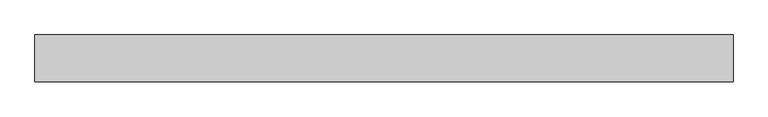
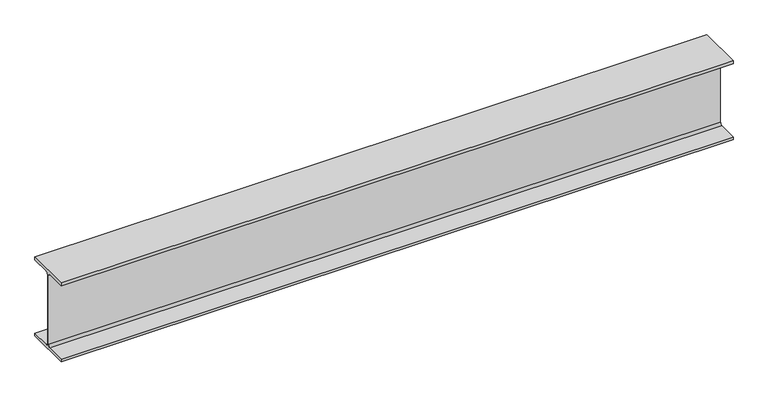
"""IFC4 building model written with IfcOpenShell, lengths in millimetres: beam geometry, Old_Steel Beam_H-KSD3502 : H_SB_ASB_H-194×150x6x9."""

from ifc_helpers import new_model, si_unit, point, frame, frame_2d, origin, place, context, project, spatial, polyline, circle_curve, trimmed, segment, composite_curve, outline, extrude, source, transform, mapped, element, save


def beam_56381f75(model_context):
    return source(origin(), model_context, "Body", "SweptSolid", [
        extrude(outline(composite_curve([segment(polyline([(82.5, -141.5), (82.5, -151.7), (-82.5, -151.7), (-82.5, -141.5), (-11.9, -141.5)]), True, "CONTINUOUS"), segment(trimmed(circle_curve(frame_2d((-11.9, -132.6)), 8.9), [point((-11.9, -141.5))], [point((-3.0, -132.6))], True, "CARTESIAN"), True, "CONTINUOUS"), segment(polyline([(-3.0, -132.6), (-3.0, 132.6)]), True, "CONTINUOUS"), segment(trimmed(circle_curve(frame_2d((-11.9, 132.6)), 8.9), [point((-3.0, 132.6))], [point((-11.9, 141.5))], True, "CARTESIAN"), True, "CONTINUOUS"), segment(polyline([(-11.9, 141.5), (-82.5, 141.5), (-82.5, 151.7), (82.5, 151.7), (82.5, 141.5), (11.9, 141.5)]), True, "CONTINUOUS"), segment(trimmed(circle_curve(frame_2d((11.9, 132.6)), 8.9), [point((11.9, 141.5))], [point((3.0, 132.6))], True, "CARTESIAN"), True, "CONTINUOUS"), segment(polyline([(3.0, 132.6), (3.0, -132.6)]), True, "CONTINUOUS"), segment(trimmed(circle_curve(frame_2d((11.9, -132.6)), 8.9), [point((3.0, -132.6))], [point((11.9, -141.5))], True, "CARTESIAN"), True, "CONTINUOUS"), segment(polyline([(11.9, -141.5), (82.5, -141.5)]), True, "CONTINUOUS")], self_intersect=False)), frame((-1200.0, 0.0, 0.0), z_axis=(1.0, 0.0, 0.0), x_axis=(0.0, 1.0, 0.0)), (0.0, 0.0, 1.0), 2448.0465428),
    ])


if __name__ == "__main__":
    model = new_model("IFC4")
    model_context = context("Model", 3, world=origin())
    ifc_project = project(units=[si_unit("LENGTHUNIT", "METRE", prefix="MILLI")], contexts=[model_context])
    site = spatial("IfcSite", under=ifc_project)
    building = spatial("IfcBuilding", under=site)
    placement = place(None, origin())
    beam_shape = beam_56381f75(model_context)
    element("IfcBeam", 1, ObjectType="Old_Steel Beam_H-KSD3502 : H_SB_ASB_H-194×150x6x9", at=placement, inside=building, context=model_context, shape_type="MappedRepresentation", body=[
        mapped(beam_shape, transform((0.0, 0.0, 0.0), x_axis=(1.0, 0.0, 0.0), y_axis=(0.0, 1.0, 0.0), z_axis=(0.0, 0.0, 1.0))),
    ])
    save(model, "model.ifc")

# Revit data of these elements
# Type "Old_Steel Beam_H-KSD3502 : H_SB_ASB_H-194×150x6x9"
#   Width = 15.0 cm
#   Web Thickness = 0.6 cm
#   Web Fillet = 1.3 cm
#   Warping Constant = 43316.0 cm⁶
#   Torsional Moment of Inertia = 8.622 cm⁴
#   Torsional Modulus = 1.0 cm³
#   Section Area = 39.01 cm²
#   Plastic Modulus weak axis = 104.0 cm³
#   Plastic Modulus strong axis = 309.0 cm³
#   Perimeter = 0.95 m²/m
#   Nominal Weight = 30.60 kgf/m
#   Moment of Inertia weak axis = 507.00 cm⁴
#   Moment of Inertia strong axis = 2690.00 cm⁴
#   Height = 19.4 cm
#   Flange Thickness = 0.9 cm
#   Elastic Modulus weak axis = 67.6 cm³
#   Elastic Modulus strong axis = 277.0 cm³
#   Centroid Vertical = 9.7 cm
#   Centroid Horizontal = 7.5 cm
#   Length [instance default] = 1.5240 m
#   Structural Material [instance default] = Steel, 45-345
#   Assembly Code = ""
# Element 1 (IfcBeam, "Old_Steel Beam_H-KSD3502 : H_SB_ASB_H-194×150x6x9")
#   Structural Material = none
# Materials
#   "Steel, 45-345": class "Metal", colour RGB 189 187 185, transparency 0, Description = "Steel 345 MPa", Cost = 0
